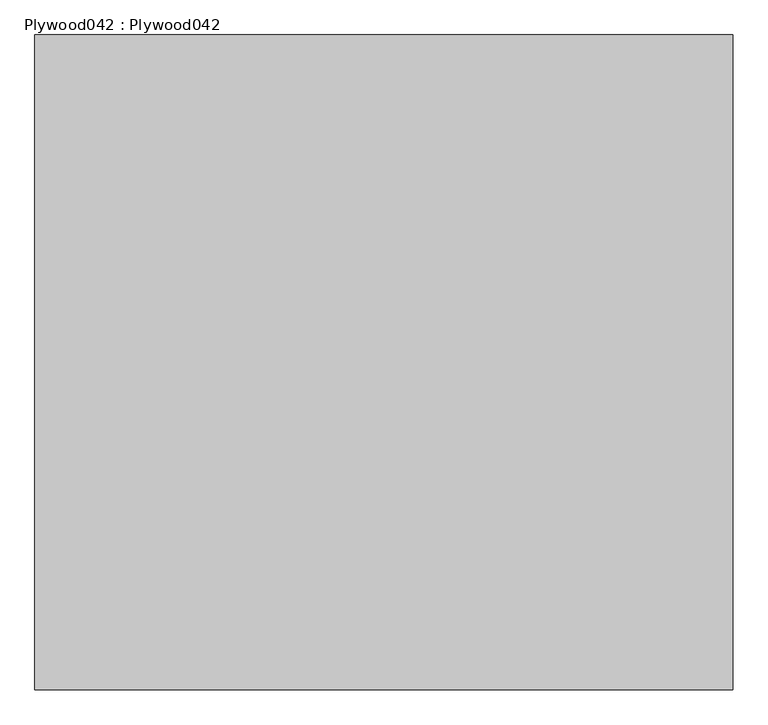
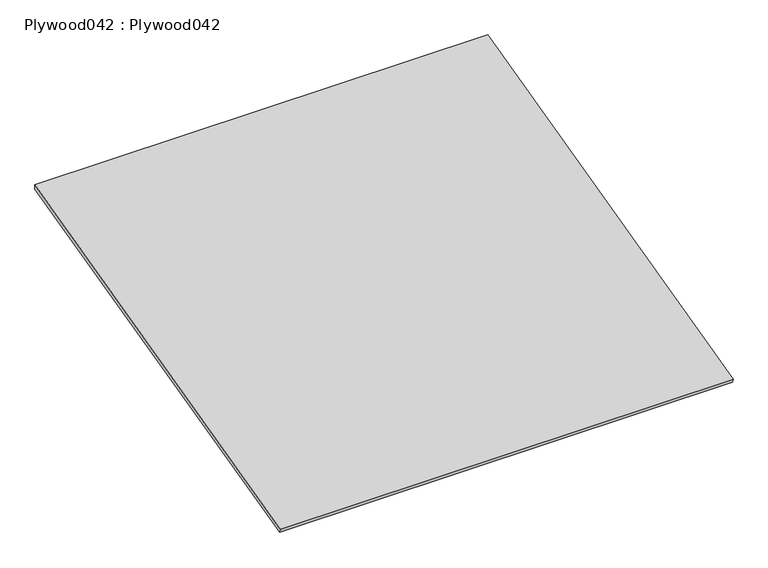
"""IFC4 building model written with IfcOpenShell, lengths in millimetres: proxy geometry, Plywood042 : Plywood042."""

import ifcopenshell
import ifcopenshell.guid

model = None  # the IFC model being written
_history = None  # IfcOwnerHistory: only IFC2X3 demands one
_inside = {}  # id of a spatial element -> (the spatial element, [elements in it])
_under = {}  # id of a project, library or spatial element -> (it, [spatial elements below it])
_declared = {}  # id of a project -> (the project, [libraries it declares])
_typed = {}  # id of a type object -> (the type object, [elements of that type])
_made_of = {}  # id of a material, layer set ... -> (it, [elements and type objects made of it])


def new_model(schema):
    """Start an empty IFC model of exactly this schema.

    Asked for "IFC4X3", IfcOpenShell would pick the latest addendum, in which some entities
    have other attributes; the version numbers below select the first issue.
    IFC2X3 requires an IfcOwnerHistory on every rooted entity: one is made here for all.
    """
    global model, _history
    if schema == "IFC4X3":
        model = ifcopenshell.file(schema_version=(4, 3, 0, 0))
    else:
        model = ifcopenshell.file(schema=schema)
    _inside.clear()
    _under.clear()
    _declared.clear()
    _typed.clear()
    _made_of.clear()
    _history = None
    if model.schema == "IFC2X3":
        org = make("IfcOrganization", Name="unknown")
        user = make(
            "IfcPersonAndOrganization",
            ThePerson=make("IfcPerson", FamilyName="unknown"),
            TheOrganization=org,
        )
        app = make(
            "IfcApplication",
            ApplicationDeveloper=org,
            Version="unknown",
            ApplicationFullName="unknown",
            ApplicationIdentifier="unknown",
        )
        _history = make(
            "IfcOwnerHistory",
            OwningUser=user,
            OwningApplication=app,
            ChangeAction="ADDED",
            CreationDate=0,
        )
    return model


def make(cls, **values):
    """One entity of the class cls with the attributes given. An attribute that is None is left unset."""
    return model.create_entity(
        cls, **{name: value for name, value in values.items() if value is not None}
    )


def rooted(cls, **values):
    """An entity with a GlobalId (a new one), such as an element, a storey or a relation."""
    return make(cls, GlobalId=ifcopenshell.guid.new(), OwnerHistory=_history, **values)


def si_unit(unit_type, name, prefix=None):
    """IfcSIUnit, for example si_unit("LENGTHUNIT", "METRE", prefix="MILLI")."""
    return make("IfcSIUnit", UnitType=unit_type, Prefix=prefix, Name=name)


def assignment(units):
    """IfcUnitAssignment: the units of a project."""
    return None if units is None else make("IfcUnitAssignment", Units=units)


def point(xyz):
    """IfcCartesianPoint."""
    return None if xyz is None else make("IfcCartesianPoint", Coordinates=xyz)


def direction(xyz):
    """IfcDirection."""
    return None if xyz is None else make("IfcDirection", DirectionRatios=xyz)


def frame(location, z_axis=None, x_axis=None):
    """IfcAxis2Placement3D, a coordinate frame: its origin and axes. An axis left out is left unset."""
    return make(
        "IfcAxis2Placement3D",
        Location=point(location),
        Axis=direction(z_axis),
        RefDirection=direction(x_axis),
    )


def origin():
    """The frame at (0, 0, 0) with its axes left unset."""
    return frame((0.0, 0.0, 0.0))


def place(relative_to, where):
    """IfcLocalPlacement: puts the frame where relative to a parent placement (None: the world)."""
    return make(
        "IfcLocalPlacement", PlacementRelTo=relative_to, RelativePlacement=where
    )


def context(
    kind, dimensions, precision=None, world=None, true_north=None, identifier=None
):
    """IfcGeometricRepresentationContext, for example the 3D "Model" context."""
    return make(
        "IfcGeometricRepresentationContext",
        ContextIdentifier=identifier,
        ContextType=kind,
        CoordinateSpaceDimension=dimensions,
        Precision=precision,
        WorldCoordinateSystem=world,
        TrueNorth=true_north,
    )


def project(units=None, contexts=None):
    """IfcProject with its units and contexts."""
    return rooted(
        "IfcProject",
        Name="project",
        RepresentationContexts=contexts,
        UnitsInContext=assignment(units),
    )


def spatial(cls, under=None, at=None, **own):
    """A site, building, storey or space (cls), placed at a placement, below another one or the project."""
    s = rooted(cls, ObjectPlacement=at, **own)
    if under is not None:
        _under.setdefault(under.id(), (under, []))[1].append(s)
    return s


def polyline(points):
    """IfcPolyline through the points."""
    return make("IfcPolyline", Points=[point(p) for p in points])


def outline(outer, holes=None, kind="AREA"):
    """IfcArbitraryClosedProfileDef: a profile drawn as a closed curve; with holes, ...WithVoids."""
    if holes is None:
        return make("IfcArbitraryClosedProfileDef", ProfileType=kind, OuterCurve=outer)
    return make(
        "IfcArbitraryProfileDefWithVoids",
        ProfileType=kind,
        OuterCurve=outer,
        InnerCurves=holes,
    )


def extrude(swept, where, along, depth):
    """IfcExtrudedAreaSolid: the profile swept, set in the frame where, extruded along a direction by depth."""
    return make(
        "IfcExtrudedAreaSolid",
        SweptArea=swept,
        Position=where,
        ExtrudedDirection=direction(along),
        Depth=depth,
    )


def shape(context_of_items, identifier, shape_type, items):
    """IfcShapeRepresentation: the items that make up one representation, for example the "Body"."""
    return make(
        "IfcShapeRepresentation",
        ContextOfItems=context_of_items,
        RepresentationIdentifier=identifier,
        RepresentationType=shape_type,
        Items=items,
    )


def source(mapping_origin, context_of_items, identifier, shape_type, items):
    """IfcRepresentationMap: a shape defined once, which mapped items show again and again."""
    return make(
        "IfcRepresentationMap",
        MappingOrigin=mapping_origin,
        MappedRepresentation=shape(context_of_items, identifier, shape_type, items),
    )


def transform(
    local_origin,
    x_axis=None,
    y_axis=None,
    z_axis=None,
    scale=None,
    scale2=None,
    scale3=None,
    uniform=True,
):
    """IfcCartesianTransformationOperator3D, or its non-uniform kind. x_axis, y_axis, z_axis: its Axis1, 2, 3."""
    if uniform:
        return make(
            "IfcCartesianTransformationOperator3D",
            Axis1=direction(x_axis),
            Axis2=direction(y_axis),
            LocalOrigin=point(local_origin),
            Scale=scale,
            Axis3=direction(z_axis),
        )
    return make(
        "IfcCartesianTransformationOperator3DnonUniform",
        Axis1=direction(x_axis),
        Axis2=direction(y_axis),
        LocalOrigin=point(local_origin),
        Scale=scale,
        Axis3=direction(z_axis),
        Scale2=scale2,
        Scale3=scale3,
    )


def mapped(mapping_source, mapping_target):
    """IfcMappedItem: shows the shape of a source again, moved by a transform."""
    return make(
        "IfcMappedItem", MappingSource=mapping_source, MappingTarget=mapping_target
    )


def made_of(thing, what):
    """Note that an element or type object is made of a material, layer set ...; save() writes the relation."""
    if what is not None:
        _made_of.setdefault(what.id(), (what, []))[1].append(thing)
    return thing


def element(
    cls,
    number,
    at=None,
    inside=None,
    cuts=None,
    type_object=None,
    material=None,
    context=None,
    identifier="Body",
    shape_type=None,
    held_by="IfcProductDefinitionShape",
    body=None,
    shapes=None,
    **own,
):
    """One element of the class cls, such as IfcWall. Its Tag is "e" and its number.

    at: its placement. inside: the storey or other place that contains it. cuts: it is an
    opening in that element (IfcRelVoidsElement). A single representation is given by context,
    identifier, shape_type and body (its items); several are given by shapes. held_by: the class
    of the entity that holds the representations. save() writes the other relations.
    """
    e = rooted(cls, Tag="e%d" % number, ObjectPlacement=at, **own)
    if body is not None:
        shapes = [shape(context, identifier, shape_type, body)]
    if shapes is not None:
        e.Representation = make(held_by, Representations=shapes)
    if inside is not None:
        _inside.setdefault(inside.id(), (inside, []))[1].append(e)
    if cuts is not None:
        rooted(
            "IfcRelVoidsElement", RelatingBuildingElement=cuts, RelatedOpeningElement=e
        )
    if type_object is not None:
        _typed.setdefault(type_object.id(), (type_object, []))[1].append(e)
    return made_of(e, material)


def aggregate(whole, parts):
    """IfcRelAggregates: a whole, such as a stair, and the parts it consists of."""
    return rooted("IfcRelAggregates", RelatingObject=whole, RelatedObjects=parts)


def save(model, path):
    """Write the relations noted so far, then the file.

    IfcRelAggregates (storeys below a building ...), IfcRelContainedInSpatialStructure (elements
    in a storey), IfcRelDefinesByType, IfcRelAssociatesMaterial and IfcRelDeclares: one each for
    every whole, place, type object, material and project.
    """
    for whole, parts in _under.values():
        aggregate(whole, parts)
    for where, things in _inside.values():
        rooted(
            "IfcRelContainedInSpatialStructure",
            RelatedElements=things,
            RelatingStructure=where,
        )
    for kind, things in _typed.values():
        rooted("IfcRelDefinesByType", RelatedObjects=things, RelatingType=kind)
    for what, things in _made_of.values():
        rooted("IfcRelAssociatesMaterial", RelatedObjects=things, RelatingMaterial=what)
    for by, libraries in _declared.values():
        rooted("IfcRelDeclares", RelatingContext=by, RelatedDefinitions=libraries)
    model.write(path)


def plywood042_plywood042_13f11387(model_context):
    return source(origin(), model_context, "Body", "SweptSolid", [
        extrude(outline(polyline([(-5217.6083572, 42802.4804791), (-5222.2286609, 42820.9616937), (-3345.9908907, 43290.0211362), (-3345.9908907, 43270.3848457), (-5217.6083572, 42802.4804791)])), frame((12383.0178845, 0.0, 0.0), z_axis=(1.0, 0.0, 0.0), x_axis=(0.0, 1.0, 0.0)), (0.0, 0.0, 1.0), 2000.0),
    ])


if __name__ == "__main__":
    model = new_model("IFC4")
    model_context = context("Model", 3, world=origin())
    ifc_project = project(units=[si_unit("LENGTHUNIT", "METRE", prefix="MILLI")], contexts=[model_context])
    site = spatial("IfcSite", under=ifc_project)
    building = spatial("IfcBuilding", under=site)
    placement = place(None, origin())
    plywood042_plywood042_shape = plywood042_plywood042_13f11387(model_context)
    element("IfcBuildingElementProxy", 1, Name="Plywood042 : Plywood042", ObjectType="Plywood042 : Plywood042", at=placement, inside=building, context=model_context, shape_type="MappedRepresentation", body=[
        mapped(plywood042_plywood042_shape, transform((0.0, 0.0, 0.0), x_axis=(1.0, 0.0, 0.0), y_axis=(0.0, 1.0, 0.0), z_axis=(0.0, 0.0, 1.0))),
    ])
    save(model, "model.ifc")

# Revit data of these elements
# Type "Plywood042 : Plywood042"
#   NameOverride = "Plywood042"
# Element 1 (IfcBuildingElementProxy, "Plywood042 : Plywood042")
#   Materials on its faces: "CDX PLYWOOD - SEE STRUCTURAL DWGS"
# Materials
#   "CDX PLYWOOD - SEE STRUCTURAL DWGS": class "Unassigned", colour RGB 177 130 114, transparency 0, Cost = 0
